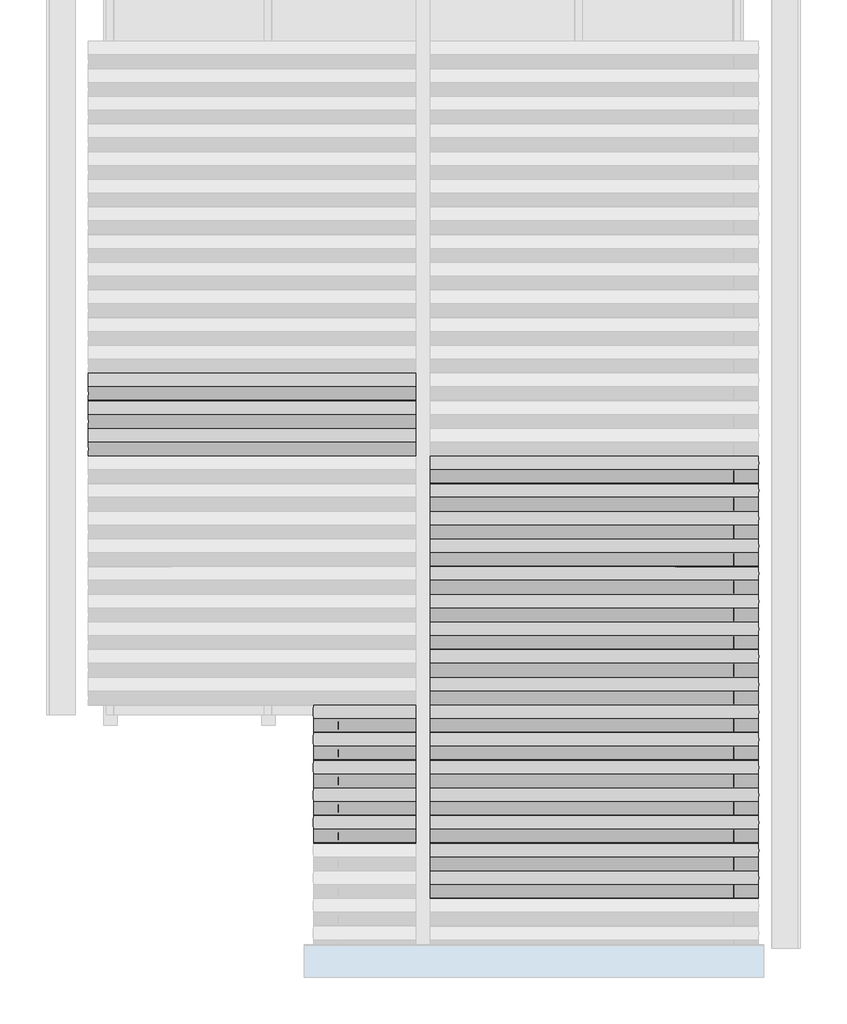
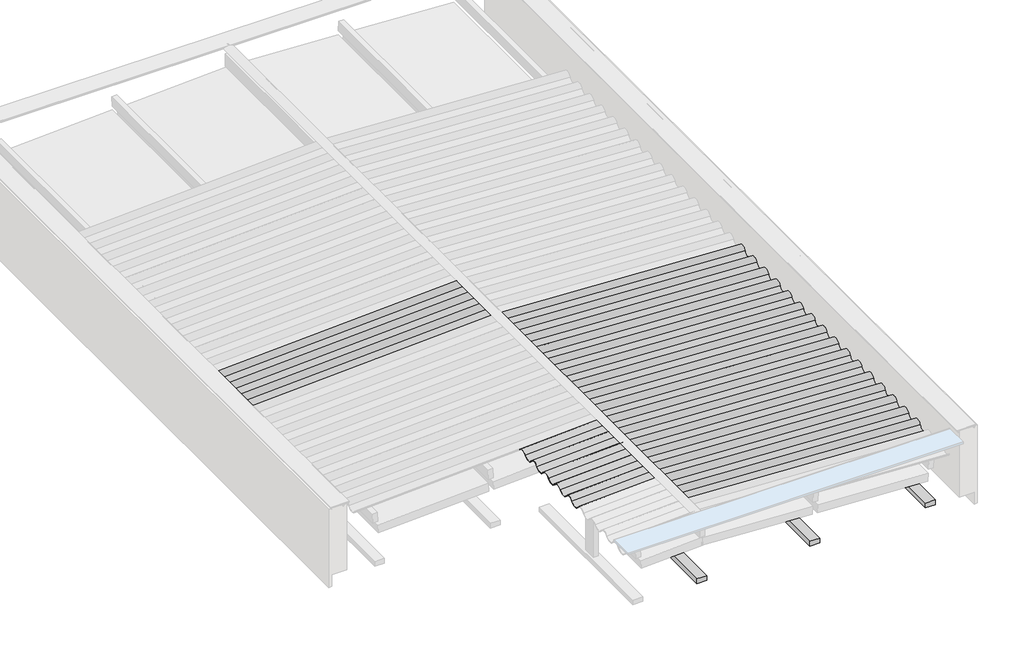
# One storey, part 2 of 4: 31 beams, 7 columns.
"""IFC4 building model written with IfcOpenShell, lengths in millimetres."""

import ifcopenshell
import ifcopenshell.guid

model = None  # the IFC model being written
_history = None  # IfcOwnerHistory: only IFC2X3 demands one
_inside = {}  # id of a spatial element -> (the spatial element, [elements in it])
_under = {}  # id of a project, library or spatial element -> (it, [spatial elements below it])
_declared = {}  # id of a project -> (the project, [libraries it declares])
_typed = {}  # id of a type object -> (the type object, [elements of that type])
_made_of = {}  # id of a material, layer set ... -> (it, [elements and type objects made of it])


def new_model(schema):
    """Start an empty IFC model of exactly this schema.

    Asked for "IFC4X3", IfcOpenShell would pick the latest addendum, in which some entities
    have other attributes; the version numbers below select the first issue.
    IFC2X3 requires an IfcOwnerHistory on every rooted entity: one is made here for all.
    """
    global model, _history
    if schema == "IFC4X3":
        model = ifcopenshell.file(schema_version=(4, 3, 0, 0))
    else:
        model = ifcopenshell.file(schema=schema)
    _inside.clear()
    _under.clear()
    _declared.clear()
    _typed.clear()
    _made_of.clear()
    _history = None
    if model.schema == "IFC2X3":
        org = make("IfcOrganization", Name="unknown")
        user = make(
            "IfcPersonAndOrganization",
            ThePerson=make("IfcPerson", FamilyName="unknown"),
            TheOrganization=org,
        )
        app = make(
            "IfcApplication",
            ApplicationDeveloper=org,
            Version="unknown",
            ApplicationFullName="unknown",
            ApplicationIdentifier="unknown",
        )
        _history = make(
            "IfcOwnerHistory",
            OwningUser=user,
            OwningApplication=app,
            ChangeAction="ADDED",
            CreationDate=0,
        )
    return model


def make(cls, **values):
    """One entity of the class cls with the attributes given. An attribute that is None is left unset."""
    return model.create_entity(
        cls, **{name: value for name, value in values.items() if value is not None}
    )


def rooted(cls, **values):
    """An entity with a GlobalId (a new one), such as an element, a storey or a relation."""
    return make(cls, GlobalId=ifcopenshell.guid.new(), OwnerHistory=_history, **values)


def si_unit(unit_type, name, prefix=None):
    """IfcSIUnit, for example si_unit("LENGTHUNIT", "METRE", prefix="MILLI")."""
    return make("IfcSIUnit", UnitType=unit_type, Prefix=prefix, Name=name)


def assignment(units):
    """IfcUnitAssignment: the units of a project."""
    return None if units is None else make("IfcUnitAssignment", Units=units)


def point(xyz):
    """IfcCartesianPoint."""
    return None if xyz is None else make("IfcCartesianPoint", Coordinates=xyz)


def direction(xyz):
    """IfcDirection."""
    return None if xyz is None else make("IfcDirection", DirectionRatios=xyz)


def frame(location, z_axis=None, x_axis=None):
    """IfcAxis2Placement3D, a coordinate frame: its origin and axes. An axis left out is left unset."""
    return make(
        "IfcAxis2Placement3D",
        Location=point(location),
        Axis=direction(z_axis),
        RefDirection=direction(x_axis),
    )


def frame_2d(location, x_axis=None):
    """IfcAxis2Placement2D, a coordinate frame in the plane: its origin and x axis."""
    return make(
        "IfcAxis2Placement2D", Location=point(location), RefDirection=direction(x_axis)
    )


def origin():
    """The frame at (0, 0, 0) with its axes left unset."""
    return frame((0.0, 0.0, 0.0))


def place(relative_to, where):
    """IfcLocalPlacement: puts the frame where relative to a parent placement (None: the world)."""
    return make(
        "IfcLocalPlacement", PlacementRelTo=relative_to, RelativePlacement=where
    )


def context(
    kind, dimensions, precision=None, world=None, true_north=None, identifier=None
):
    """IfcGeometricRepresentationContext, for example the 3D "Model" context."""
    return make(
        "IfcGeometricRepresentationContext",
        ContextIdentifier=identifier,
        ContextType=kind,
        CoordinateSpaceDimension=dimensions,
        Precision=precision,
        WorldCoordinateSystem=world,
        TrueNorth=true_north,
    )


def project(units=None, contexts=None):
    """IfcProject with its units and contexts."""
    return rooted(
        "IfcProject",
        Name="project",
        RepresentationContexts=contexts,
        UnitsInContext=assignment(units),
    )


def spatial(cls, under=None, at=None, **own):
    """A site, building, storey or space (cls), placed at a placement, below another one or the project."""
    s = rooted(cls, ObjectPlacement=at, **own)
    if under is not None:
        _under.setdefault(under.id(), (under, []))[1].append(s)
    return s


def polyline(points):
    """IfcPolyline through the points."""
    return make("IfcPolyline", Points=[point(p) for p in points])


def circle_curve(where, radius):
    """IfcCircle in the frame where."""
    return make("IfcCircle", Position=where, Radius=radius)


def trimmed(basis, trim1, trim2, sense, master):
    """IfcTrimmedCurve: the piece of a basis curve between two trims."""
    return make(
        "IfcTrimmedCurve",
        BasisCurve=basis,
        Trim1=trim1,
        Trim2=trim2,
        SenseAgreement=sense,
        MasterRepresentation=master,
    )


def segment(curve, same_sense, transition):
    """IfcCompositeCurveSegment."""
    return make(
        "IfcCompositeCurveSegment",
        Transition=transition,
        SameSense=same_sense,
        ParentCurve=curve,
    )


def composite_curve(segments, self_intersect=None):
    """IfcCompositeCurve: segments joined end to end."""
    return make("IfcCompositeCurve", Segments=segments, SelfIntersect=self_intersect)


def outline(outer, holes=None, kind="AREA"):
    """IfcArbitraryClosedProfileDef: a profile drawn as a closed curve; with holes, ...WithVoids."""
    if holes is None:
        return make("IfcArbitraryClosedProfileDef", ProfileType=kind, OuterCurve=outer)
    return make(
        "IfcArbitraryProfileDefWithVoids",
        ProfileType=kind,
        OuterCurve=outer,
        InnerCurves=holes,
    )


def extrude(swept, where, along, depth):
    """IfcExtrudedAreaSolid: the profile swept, set in the frame where, extruded along a direction by depth."""
    return make(
        "IfcExtrudedAreaSolid",
        SweptArea=swept,
        Position=where,
        ExtrudedDirection=direction(along),
        Depth=depth,
    )


def shape(context_of_items, identifier, shape_type, items):
    """IfcShapeRepresentation: the items that make up one representation, for example the "Body"."""
    return make(
        "IfcShapeRepresentation",
        ContextOfItems=context_of_items,
        RepresentationIdentifier=identifier,
        RepresentationType=shape_type,
        Items=items,
    )


def source(mapping_origin, context_of_items, identifier, shape_type, items):
    """IfcRepresentationMap: a shape defined once, which mapped items show again and again."""
    return make(
        "IfcRepresentationMap",
        MappingOrigin=mapping_origin,
        MappedRepresentation=shape(context_of_items, identifier, shape_type, items),
    )


def transform(
    local_origin,
    x_axis=None,
    y_axis=None,
    z_axis=None,
    scale=None,
    scale2=None,
    scale3=None,
    uniform=True,
):
    """IfcCartesianTransformationOperator3D, or its non-uniform kind. x_axis, y_axis, z_axis: its Axis1, 2, 3."""
    if uniform:
        return make(
            "IfcCartesianTransformationOperator3D",
            Axis1=direction(x_axis),
            Axis2=direction(y_axis),
            LocalOrigin=point(local_origin),
            Scale=scale,
            Axis3=direction(z_axis),
        )
    return make(
        "IfcCartesianTransformationOperator3DnonUniform",
        Axis1=direction(x_axis),
        Axis2=direction(y_axis),
        LocalOrigin=point(local_origin),
        Scale=scale,
        Axis3=direction(z_axis),
        Scale2=scale2,
        Scale3=scale3,
    )


def mapped(mapping_source, mapping_target):
    """IfcMappedItem: shows the shape of a source again, moved by a transform."""
    return make(
        "IfcMappedItem", MappingSource=mapping_source, MappingTarget=mapping_target
    )


def made_of(thing, what):
    """Note that an element or type object is made of a material, layer set ...; save() writes the relation."""
    if what is not None:
        _made_of.setdefault(what.id(), (what, []))[1].append(thing)
    return thing


def element(
    cls,
    number,
    at=None,
    inside=None,
    cuts=None,
    type_object=None,
    material=None,
    context=None,
    identifier="Body",
    shape_type=None,
    held_by="IfcProductDefinitionShape",
    body=None,
    shapes=None,
    **own,
):
    """One element of the class cls, such as IfcWall. Its Tag is "e" and its number.

    at: its placement. inside: the storey or other place that contains it. cuts: it is an
    opening in that element (IfcRelVoidsElement). A single representation is given by context,
    identifier, shape_type and body (its items); several are given by shapes. held_by: the class
    of the entity that holds the representations. save() writes the other relations.
    """
    e = rooted(cls, Tag="e%d" % number, ObjectPlacement=at, **own)
    if body is not None:
        shapes = [shape(context, identifier, shape_type, body)]
    if shapes is not None:
        e.Representation = make(held_by, Representations=shapes)
    if inside is not None:
        _inside.setdefault(inside.id(), (inside, []))[1].append(e)
    if cuts is not None:
        rooted(
            "IfcRelVoidsElement", RelatingBuildingElement=cuts, RelatedOpeningElement=e
        )
    if type_object is not None:
        _typed.setdefault(type_object.id(), (type_object, []))[1].append(e)
    return made_of(e, material)


def aggregate(whole, parts):
    """IfcRelAggregates: a whole, such as a stair, and the parts it consists of."""
    return rooted("IfcRelAggregates", RelatingObject=whole, RelatedObjects=parts)


def save(model, path):
    """Write the relations noted so far, then the file.

    IfcRelAggregates (storeys below a building ...), IfcRelContainedInSpatialStructure (elements
    in a storey), IfcRelDefinesByType, IfcRelAssociatesMaterial and IfcRelDeclares: one each for
    every whole, place, type object, material and project.
    """
    for whole, parts in _under.values():
        aggregate(whole, parts)
    for where, things in _inside.values():
        rooted(
            "IfcRelContainedInSpatialStructure",
            RelatedElements=things,
            RelatingStructure=where,
        )
    for kind, things in _typed.values():
        rooted("IfcRelDefinesByType", RelatedObjects=things, RelatingType=kind)
    for what, things in _made_of.values():
        rooted("IfcRelAssociatesMaterial", RelatedObjects=things, RelatingMaterial=what)
    for by, libraries in _declared.values():
        rooted("IfcRelDeclares", RelatingContext=by, RelatedDefinitions=libraries)
    model.write(path)


def column_f3930958(model_context):
    return source(origin(), model_context, "Body", "SweptSolid", [
        extrude(outline(polyline([(30.0, 80.0), (30.0, -80.0), (-30.0, -80.0), (-30.0, 80.0), (30.0, 80.0)])), frame((0.0, 0.0, 4460.0), z_axis=(0.0, 0.0, 1.0), x_axis=(1.0, 0.0, 0.0)), (0.0, 0.0, 1.0), 522.9),
    ])


def column_4d3918cc(model_context):
    return source(origin(), model_context, "Body", "SweptSolid", [
        extrude(outline(polyline([(30.0, 80.0), (30.0, -80.0), (-30.0, -80.0), (-30.0, 80.0), (30.0, 80.0)])), frame((0.0, 0.0, 4460.0), z_axis=(0.0, 0.0, 1.0), x_axis=(1.0, 0.0, 0.0)), (0.0, 0.0, 1.0), 426.9),
    ])


def column_924cc83b(model_context):
    return source(origin(), model_context, "Body", "SweptSolid", [
        extrude(outline(polyline([(30.0, 80.0), (30.0, -80.0), (-30.0, -80.0), (-30.0, 80.0), (30.0, 80.0)])), frame((0.0, 0.0, 4460.0), z_axis=(0.0, 0.0, 1.0), x_axis=(1.0, 0.0, 0.0)), (0.0, 0.0, 1.0), 497.0),
    ])


model = new_model("IFC4")

# Units and contexts
model_context = context("Model", 3, world=origin())
ifc_project = project(units=[si_unit("LENGTHUNIT", "METRE", prefix="MILLI")], contexts=[model_context])

# Site, building, storey
site = spatial("IfcSite", under=ifc_project)
building = spatial("IfcBuilding", under=site)
storey = spatial("IfcBuildingStorey", under=building, Name="COB. SALA ESTAR", Elevation=4400.0)

# Beams
placement = place(None, origin())
element("IfcBeam", 1, ObjectType="Madeira de lei : Berço 6x12cm", at=placement, inside=storey, context=model_context, shape_type="SweptSolid", body=[
    extrude(outline(polyline([(-3400.781307, -376.0699847), (-3280.781307, -376.0699847), (-3280.781307, -2376.0699847), (-3400.781307, -2376.0699847), (-3400.781307, -376.0699847)])), frame((0.0, 0.0, 4400.0), z_axis=(0.0, 0.0, 1.0), x_axis=(1.0, 0.0, 0.0)), (0.0, 0.0, 1.0), 60.0),
])
element("IfcBeam", 2, ObjectType="Madeira de lei : Berço 6x12cm", at=placement, inside=storey, context=model_context, shape_type="SweptSolid", body=[
    extrude(outline(polyline([(-3400.781307, -2376.0699847), (-3280.781307, -2376.0699847), (-3280.781307, -4336.0699847), (-3400.781307, -4336.0699847), (-3400.781307, -2376.0699847)])), frame((0.0, 0.0, 4400.0), z_axis=(0.0, 0.0, 1.0), x_axis=(1.0, 0.0, 0.0)), (0.0, 0.0, 1.0), 60.0),
])
element("IfcBeam", 3, ObjectType="Madeira de lei : Berço 6x12cm", at=placement, inside=storey, context=model_context, shape_type="SweptSolid", body=[
    extrude(outline(polyline([(-2032.4438771, -376.0699847), (-1912.4438771, -376.0699847), (-1912.4438771, -2376.0699847), (-2032.4438771, -2376.0699847), (-2032.4438771, -376.0699847)])), frame((0.0, 0.0, 4400.0), z_axis=(0.0, 0.0, 1.0), x_axis=(1.0, 0.0, 0.0)), (0.0, 0.0, 1.0), 60.0),
])
element("IfcBeam", 4, ObjectType="Madeira de lei : Berço 6x12cm", at=placement, inside=storey, context=model_context, shape_type="SweptSolid", body=[
    extrude(outline(polyline([(-2032.4438771, -2376.0699847), (-1912.4438771, -2376.0699847), (-1912.4438771, -4336.0699847), (-2032.4438771, -4336.0699847), (-2032.4438771, -2376.0699847)])), frame((0.0, 0.0, 4400.0), z_axis=(0.0, 0.0, 1.0), x_axis=(1.0, 0.0, 0.0)), (0.0, 0.0, 1.0), 60.0),
])
element("IfcBeam", 5, ObjectType="Madeira de lei : Berço 6x12cm", at=placement, inside=storey, context=model_context, shape_type="SweptSolid", body=[
    extrude(outline(polyline([(-634.1438771, -376.0699847), (-514.1438771, -376.0699847), (-514.1438771, -2376.0699847), (-634.1438771, -2376.0699847), (-634.1438771, -376.0699847)])), frame((0.0, 0.0, 4400.0), z_axis=(0.0, 0.0, 1.0), x_axis=(1.0, 0.0, 0.0)), (0.0, 0.0, 1.0), 60.0),
])
element("IfcBeam", 6, ObjectType="Madeira de lei : Berço 6x12cm", at=placement, inside=storey, context=model_context, shape_type="SweptSolid", body=[
    extrude(outline(polyline([(-634.1438771, -2376.0699847), (-514.1438771, -2376.0699847), (-514.1438771, -4336.0699847), (-634.1438771, -4336.0699847), (-634.1438771, -2376.0699847)])), frame((0.0, 0.0, 4400.0), z_axis=(0.0, 0.0, 1.0), x_axis=(1.0, 0.0, 0.0)), (0.0, 0.0, 1.0), 60.0),
])
element("IfcBeam", 7, ObjectType="Madeira de lei : Berço 6x12cm", at=placement, inside=storey, context=model_context, shape_type="SweptSolid", body=[
    extrude(outline(polyline([(-6167.4187368, 1623.9300153), (-6047.4187368, 1623.9300153), (-6047.4187368, -376.0699847), (-6167.4187368, -376.0699847), (-6167.4187368, 1623.9300153)])), frame((0.0, 0.0, 4400.0), z_axis=(0.0, 0.0, 1.0), x_axis=(1.0, 0.0, 0.0)), (0.0, 0.0, 1.0), 60.0),
])
element("IfcBeam", 8, ObjectType="Telha Ondulada : Fibrocimento", at=placement, inside=storey, context=model_context, shape_type="SweptSolid", body=[
    extrude(outline(composite_curve([segment(trimmed(circle_curve(frame_2d((-58.7002978, -53.2060538)), 66.7939461), [point((-29.3501489, 6.7939462))], [point((-29.3501489, -113.2060538))], False, "CARTESIAN"), True, "CONTINUOUS"), segment(polyline([(-29.3501489, -113.2060538), (-31.5472154, -108.7146288)]), True, "CONTINUOUS"), segment(trimmed(circle_curve(frame_2d((-58.7002978, -53.2060538)), 61.7939461), [point((-31.5472154, -108.7146288))], [point((-31.5472154, 2.3025211))], True, "CARTESIAN"), True, "CONTINUOUS"), segment(trimmed(circle_curve(frame_2d((0.0, 66.7939462)), 71.7939461), [point((-31.5472154, 2.3025211))], [point((-31.5472154, 131.2853712))], False, "CARTESIAN"), True, "CONTINUOUS"), segment(polyline([(-31.5472154, 131.2853712), (-29.3501489, 126.7939462)]), True, "CONTINUOUS"), segment(trimmed(circle_curve(frame_2d((0.0, 66.7939462)), 66.7939461), [point((-29.3501489, 126.7939462))], [point((-29.3501489, 6.7939462))], True, "CARTESIAN"), True, "CONTINUOUS")], self_intersect=False)), frame((-4311.894473, -3289.673052, 5167.7128806), z_axis=(0.9987523388778448, 0.0, 0.049937616943891816), x_axis=(-0.049937616943891816, 0.0, 0.9987523388778448)), (0.0, 0.0, 1.0), 967.7366024),
])
element("IfcBeam", 9, ObjectType="Telha Ondulada : Fibrocimento", at=placement, inside=storey, context=model_context, shape_type="SweptSolid", body=[
    extrude(outline(composite_curve([segment(trimmed(circle_curve(frame_2d((-58.7002978, -53.2060538)), 66.7939461), [point((-29.3501489, 6.7939462))], [point((-29.3501489, -113.2060538))], False, "CARTESIAN"), True, "CONTINUOUS"), segment(polyline([(-29.3501489, -113.2060538), (-31.5472154, -108.7146288)]), True, "CONTINUOUS"), segment(trimmed(circle_curve(frame_2d((-58.7002978, -53.2060538)), 61.7939461), [point((-31.5472154, -108.7146288))], [point((-31.5472154, 2.3025211))], True, "CARTESIAN"), True, "CONTINUOUS"), segment(trimmed(circle_curve(frame_2d((0.0, 66.7939462)), 71.7939461), [point((-31.5472154, 2.3025211))], [point((-31.5472154, 131.2853712))], False, "CARTESIAN"), True, "CONTINUOUS"), segment(polyline([(-31.5472154, 131.2853712), (-29.3501489, 126.7939462)]), True, "CONTINUOUS"), segment(trimmed(circle_curve(frame_2d((0.0, 66.7939462)), 66.7939461), [point((-29.3501489, 126.7939462))], [point((-29.3501489, 6.7939462))], True, "CARTESIAN"), True, "CONTINUOUS")], self_intersect=False)), frame((-4311.894473, -3045.173052, 5167.7128806), z_axis=(0.9987523388778448, 0.0, 0.049937616943891816), x_axis=(-0.049937616943891816, 0.0, 0.9987523388778448)), (0.0, 0.0, 1.0), 967.7366024),
])
element("IfcBeam", 10, ObjectType="Telha Ondulada : Fibrocimento", at=placement, inside=storey, context=model_context, shape_type="SweptSolid", body=[
    extrude(outline(composite_curve([segment(trimmed(circle_curve(frame_2d((-58.7002978, -53.2060538)), 66.7939461), [point((-29.3501489, 6.7939462))], [point((-29.3501489, -113.2060538))], False, "CARTESIAN"), True, "CONTINUOUS"), segment(polyline([(-29.3501489, -113.2060538), (-31.5472154, -108.7146288)]), True, "CONTINUOUS"), segment(trimmed(circle_curve(frame_2d((-58.7002978, -53.2060538)), 61.7939461), [point((-31.5472154, -108.7146288))], [point((-31.5472154, 2.3025211))], True, "CARTESIAN"), True, "CONTINUOUS"), segment(trimmed(circle_curve(frame_2d((0.0, 66.7939462)), 71.7939461), [point((-31.5472154, 2.3025211))], [point((-31.5472154, 131.2853712))], False, "CARTESIAN"), True, "CONTINUOUS"), segment(polyline([(-31.5472154, 131.2853712), (-29.3501489, 126.7939462)]), True, "CONTINUOUS"), segment(trimmed(circle_curve(frame_2d((0.0, 66.7939462)), 66.7939461), [point((-29.3501489, 126.7939462))], [point((-29.3501489, 6.7939462))], True, "CARTESIAN"), True, "CONTINUOUS")], self_intersect=False)), frame((-4311.894473, -2800.673052, 5167.7128806), z_axis=(0.9987523388778448, 0.0, 0.049937616943891844), x_axis=(-0.049937616943891844, 0.0, 0.9987523388778448)), (0.0, 0.0, 1.0), 967.7366024),
])
element("IfcBeam", 11, ObjectType="Telha Ondulada : Fibrocimento", at=placement, inside=storey, context=model_context, shape_type="SweptSolid", body=[
    extrude(outline(composite_curve([segment(trimmed(circle_curve(frame_2d((-58.7002978, -53.2060538)), 66.7939461), [point((-29.3501489, 6.7939462))], [point((-29.3501489, -113.2060538))], False, "CARTESIAN"), True, "CONTINUOUS"), segment(polyline([(-29.3501489, -113.2060538), (-31.5472154, -108.7146288)]), True, "CONTINUOUS"), segment(trimmed(circle_curve(frame_2d((-58.7002978, -53.2060538)), 61.7939461), [point((-31.5472154, -108.7146288))], [point((-31.5472154, 2.3025211))], True, "CARTESIAN"), True, "CONTINUOUS"), segment(trimmed(circle_curve(frame_2d((0.0, 66.7939462)), 71.7939461), [point((-31.5472154, 2.3025211))], [point((-31.5472154, 131.2853712))], False, "CARTESIAN"), True, "CONTINUOUS"), segment(polyline([(-31.5472154, 131.2853712), (-29.3501489, 126.7939462)]), True, "CONTINUOUS"), segment(trimmed(circle_curve(frame_2d((0.0, 66.7939462)), 66.7939461), [point((-29.3501489, 126.7939462))], [point((-29.3501489, 6.7939462))], True, "CARTESIAN"), True, "CONTINUOUS")], self_intersect=False)), frame((-4311.894473, -2556.173052, 5167.7128806), z_axis=(0.9987523388778448, 0.0, 0.049937616943891816), x_axis=(-0.049937616943891816, 0.0, 0.9987523388778448)), (0.0, 0.0, 1.0), 967.7366024),
])
element("IfcBeam", 12, ObjectType="Telha Ondulada : Fibrocimento", at=placement, inside=storey, context=model_context, shape_type="SweptSolid", body=[
    extrude(outline(composite_curve([segment(trimmed(circle_curve(frame_2d((-58.7002978, -53.2060538)), 66.7939461), [point((-29.3501489, 6.7939462))], [point((-29.3501489, -113.2060538))], False, "CARTESIAN"), True, "CONTINUOUS"), segment(polyline([(-29.3501489, -113.2060538), (-31.5472154, -108.7146288)]), True, "CONTINUOUS"), segment(trimmed(circle_curve(frame_2d((-58.7002978, -53.2060538)), 61.7939461), [point((-31.5472154, -108.7146288))], [point((-31.5472154, 2.3025211))], True, "CARTESIAN"), True, "CONTINUOUS"), segment(trimmed(circle_curve(frame_2d((0.0, 66.7939462)), 71.7939461), [point((-31.5472154, 2.3025211))], [point((-31.5472154, 131.2853712))], False, "CARTESIAN"), True, "CONTINUOUS"), segment(polyline([(-31.5472154, 131.2853712), (-29.3501489, 126.7939462)]), True, "CONTINUOUS"), segment(trimmed(circle_curve(frame_2d((0.0, 66.7939462)), 66.7939461), [point((-29.3501489, 126.7939462))], [point((-29.3501489, 6.7939462))], True, "CARTESIAN"), True, "CONTINUOUS")], self_intersect=False)), frame((-4311.894473, -2311.673052, 5167.7128806), z_axis=(0.9987523388778448, 0.0, 0.04993761694389179), x_axis=(-0.04993761694389179, 0.0, 0.9987523388778448)), (0.0, 0.0, 1.0), 967.7366024),
])
element("IfcBeam", 13, ObjectType="Telha Ondulada : Fibrocimento", at=placement, inside=storey, context=model_context, shape_type="SweptSolid", body=[
    extrude(outline(composite_curve([segment(trimmed(circle_curve(frame_2d((-58.7002978, -53.2060538)), 66.7939461), [point((-29.3501488, 6.7939462))], [point((-29.3501488, -113.2060538))], False, "CARTESIAN"), True, "CONTINUOUS"), segment(polyline([(-29.3501488, -113.2060538), (-31.5472154, -108.7146288)]), True, "CONTINUOUS"), segment(trimmed(circle_curve(frame_2d((-58.7002978, -53.2060538)), 61.7939461), [point((-31.5472154, -108.7146288))], [point((-31.5472154, 2.3025211))], True, "CARTESIAN"), True, "CONTINUOUS"), segment(trimmed(circle_curve(frame_2d((0.0, 66.7939462)), 71.7939461), [point((-31.5472154, 2.3025211))], [point((-31.5472154, 131.2853712))], False, "CARTESIAN"), True, "CONTINUOUS"), segment(polyline([(-31.5472154, 131.2853712), (-29.3501488, 126.7939462)]), True, "CONTINUOUS"), segment(trimmed(circle_curve(frame_2d((0.0, 66.7939462)), 66.7939461), [point((-29.3501488, 126.7939462))], [point((-29.3501488, 6.7939462))], True, "CARTESIAN"), True, "CONTINUOUS")], self_intersect=False)), frame((-6303.6781287, 133.326948, 5068.1236978), z_axis=(0.9987523388778448, 0.0, 0.049937616943891344), x_axis=(-0.049937616943891344, 0.0, 0.9987523388778448)), (0.0, 0.0, 1.0), 2962.0084336),
])
element("IfcBeam", 14, ObjectType="Telha Ondulada : Fibrocimento", at=placement, inside=storey, context=model_context, shape_type="SweptSolid", body=[
    extrude(outline(composite_curve([segment(trimmed(circle_curve(frame_2d((-58.7002978, -53.2060538)), 66.7939461), [point((-29.3501488, 6.7939462))], [point((-29.3501488, -113.2060538))], False, "CARTESIAN"), True, "CONTINUOUS"), segment(polyline([(-29.3501488, -113.2060538), (-31.5472154, -108.7146288)]), True, "CONTINUOUS"), segment(trimmed(circle_curve(frame_2d((-58.7002978, -53.2060538)), 61.7939461), [point((-31.5472154, -108.7146288))], [point((-31.5472154, 2.3025211))], True, "CARTESIAN"), True, "CONTINUOUS"), segment(trimmed(circle_curve(frame_2d((0.0, 66.7939462)), 71.7939461), [point((-31.5472154, 2.3025211))], [point((-31.5472154, 131.2853712))], False, "CARTESIAN"), True, "CONTINUOUS"), segment(polyline([(-31.5472154, 131.2853712), (-29.3501488, 126.7939462)]), True, "CONTINUOUS"), segment(trimmed(circle_curve(frame_2d((0.0, 66.7939462)), 66.7939461), [point((-29.3501488, 126.7939462))], [point((-29.3501488, 6.7939462))], True, "CARTESIAN"), True, "CONTINUOUS")], self_intersect=False)), frame((-6303.6781287, 377.826948, 5068.1236978), z_axis=(0.9987523388778449, 0.0, 0.049937616943891365), x_axis=(-0.049937616943891365, 0.0, 0.9987523388778449)), (0.0, 0.0, 1.0), 2962.0084336),
])
element("IfcBeam", 15, ObjectType="Telha Ondulada : Fibrocimento", at=placement, inside=storey, context=model_context, shape_type="SweptSolid", body=[
    extrude(outline(composite_curve([segment(trimmed(circle_curve(frame_2d((-58.7002978, -53.2060538)), 66.7939461), [point((-29.3501488, 6.7939462))], [point((-29.3501488, -113.2060538))], False, "CARTESIAN"), True, "CONTINUOUS"), segment(polyline([(-29.3501488, -113.2060538), (-31.5472154, -108.7146288)]), True, "CONTINUOUS"), segment(trimmed(circle_curve(frame_2d((-58.7002978, -53.2060538)), 61.7939461), [point((-31.5472154, -108.7146288))], [point((-31.5472154, 2.3025211))], True, "CARTESIAN"), True, "CONTINUOUS"), segment(trimmed(circle_curve(frame_2d((0.0, 66.7939462)), 71.7939461), [point((-31.5472154, 2.3025211))], [point((-31.5472154, 131.2853712))], False, "CARTESIAN"), True, "CONTINUOUS"), segment(polyline([(-31.5472154, 131.2853712), (-29.3501488, 126.7939462)]), True, "CONTINUOUS"), segment(trimmed(circle_curve(frame_2d((0.0, 66.7939462)), 66.7939461), [point((-29.3501488, 126.7939462))], [point((-29.3501488, 6.7939462))], True, "CARTESIAN"), True, "CONTINUOUS")], self_intersect=False)), frame((-6303.6781287, 622.326948, 5068.1236978), z_axis=(0.9987523388778448, 0.0, 0.04993761694389136), x_axis=(-0.04993761694389136, 0.0, 0.9987523388778448)), (0.0, 0.0, 1.0), 2962.0084336),
])
element("IfcBeam", 16, ObjectType="Telha Ondulada : Fibrocimento", at=placement, inside=storey, context=model_context, shape_type="SweptSolid", body=[
    extrude(outline(composite_curve([segment(trimmed(circle_curve(frame_2d((0.0, 66.7939462)), 66.7939461), [point((29.3501488, 6.7939462))], [point((29.3501488, 126.7939462))], True, "CARTESIAN"), True, "CONTINUOUS"), segment(polyline([(29.3501488, 126.7939462), (31.5472154, 131.2853712)]), True, "CONTINUOUS"), segment(trimmed(circle_curve(frame_2d((0.0, 66.7939462)), 71.7939461), [point((31.5472154, 131.2853712))], [point((31.5472154, 2.3025211))], False, "CARTESIAN"), True, "CONTINUOUS"), segment(trimmed(circle_curve(frame_2d((58.7002978, -53.2060538)), 61.7939461), [point((31.5472154, 2.3025211))], [point((31.5472154, -108.7146288))], True, "CARTESIAN"), True, "CONTINUOUS"), segment(polyline([(31.5472154, -108.7146288), (29.3501488, -113.2060538)]), True, "CONTINUOUS"), segment(trimmed(circle_curve(frame_2d((58.7002978, -53.2060538)), 66.7939461), [point((29.3501488, -113.2060538))], [point((29.3501488, 6.7939462))], False, "CARTESIAN"), True, "CONTINUOUS")], self_intersect=False)), frame((-377.8844852, -3778.673052, 5068.1236978), z_axis=(-0.9987523388778448, 0.0, 0.049937616943891455), x_axis=(-0.049937616943891455, 0.0, -0.9987523388778448)), (0.0, 0.0, 1.0), 2962.0084336),
])
element("IfcBeam", 17, ObjectType="Telha Ondulada : Fibrocimento", at=placement, inside=storey, context=model_context, shape_type="SweptSolid", body=[
    extrude(outline(composite_curve([segment(trimmed(circle_curve(frame_2d((0.0, 66.7939462)), 66.7939461), [point((29.3501488, 6.7939462))], [point((29.3501488, 126.7939462))], True, "CARTESIAN"), True, "CONTINUOUS"), segment(polyline([(29.3501488, 126.7939462), (31.5472154, 131.2853712)]), True, "CONTINUOUS"), segment(trimmed(circle_curve(frame_2d((0.0, 66.7939462)), 71.7939461), [point((31.5472154, 131.2853712))], [point((31.5472154, 2.3025211))], False, "CARTESIAN"), True, "CONTINUOUS"), segment(trimmed(circle_curve(frame_2d((58.7002978, -53.2060538)), 61.7939461), [point((31.5472154, 2.3025211))], [point((31.5472154, -108.7146288))], True, "CARTESIAN"), True, "CONTINUOUS"), segment(polyline([(31.5472154, -108.7146288), (29.3501488, -113.2060538)]), True, "CONTINUOUS"), segment(trimmed(circle_curve(frame_2d((58.7002978, -53.2060538)), 66.7939461), [point((29.3501488, -113.2060538))], [point((29.3501488, 6.7939462))], False, "CARTESIAN"), True, "CONTINUOUS")], self_intersect=False)), frame((-377.8844852, -3534.173052, 5068.1236978), z_axis=(-0.9987523388778448, 0.0, 0.049937616943891455), x_axis=(-0.049937616943891455, 0.0, -0.9987523388778448)), (0.0, 0.0, 1.0), 2962.0084336),
])
element("IfcBeam", 18, ObjectType="Telha Ondulada : Fibrocimento", at=placement, inside=storey, context=model_context, shape_type="SweptSolid", body=[
    extrude(outline(composite_curve([segment(trimmed(circle_curve(frame_2d((0.0, 66.7939462)), 66.7939461), [point((29.3501488, 6.7939462))], [point((29.3501488, 126.7939462))], True, "CARTESIAN"), True, "CONTINUOUS"), segment(polyline([(29.3501488, 126.7939462), (31.5472154, 131.2853712)]), True, "CONTINUOUS"), segment(trimmed(circle_curve(frame_2d((0.0, 66.7939462)), 71.7939461), [point((31.5472154, 131.2853712))], [point((31.5472154, 2.3025211))], False, "CARTESIAN"), True, "CONTINUOUS"), segment(trimmed(circle_curve(frame_2d((58.7002978, -53.2060538)), 61.7939461), [point((31.5472154, 2.3025211))], [point((31.5472154, -108.7146288))], True, "CARTESIAN"), True, "CONTINUOUS"), segment(polyline([(31.5472154, -108.7146288), (29.3501488, -113.2060538)]), True, "CONTINUOUS"), segment(trimmed(circle_curve(frame_2d((58.7002978, -53.2060538)), 66.7939461), [point((29.3501488, -113.2060538))], [point((29.3501488, 6.7939462))], False, "CARTESIAN"), True, "CONTINUOUS")], self_intersect=False)), frame((-377.8844852, -3289.673052, 5068.1236978), z_axis=(-0.9987523388778448, 0.0, 0.049937616943891455), x_axis=(-0.049937616943891455, 0.0, -0.9987523388778448)), (0.0, 0.0, 1.0), 2962.0084336),
])
element("IfcBeam", 19, ObjectType="Telha Ondulada : Fibrocimento", at=placement, inside=storey, context=model_context, shape_type="SweptSolid", body=[
    extrude(outline(composite_curve([segment(trimmed(circle_curve(frame_2d((0.0, 66.7939462)), 66.7939461), [point((29.3501488, 6.7939462))], [point((29.3501488, 126.7939462))], True, "CARTESIAN"), True, "CONTINUOUS"), segment(polyline([(29.3501488, 126.7939462), (31.5472154, 131.2853712)]), True, "CONTINUOUS"), segment(trimmed(circle_curve(frame_2d((0.0, 66.7939462)), 71.7939461), [point((31.5472154, 131.2853712))], [point((31.5472154, 2.3025211))], False, "CARTESIAN"), True, "CONTINUOUS"), segment(trimmed(circle_curve(frame_2d((58.7002978, -53.2060538)), 61.7939461), [point((31.5472154, 2.3025211))], [point((31.5472154, -108.7146288))], True, "CARTESIAN"), True, "CONTINUOUS"), segment(polyline([(31.5472154, -108.7146288), (29.3501488, -113.2060538)]), True, "CONTINUOUS"), segment(trimmed(circle_curve(frame_2d((58.7002978, -53.2060538)), 66.7939461), [point((29.3501488, -113.2060538))], [point((29.3501488, 6.7939462))], False, "CARTESIAN"), True, "CONTINUOUS")], self_intersect=False)), frame((-377.8844852, -3045.173052, 5068.1236978), z_axis=(-0.9987523388778448, 0.0, 0.049937616943891455), x_axis=(-0.049937616943891455, 0.0, -0.9987523388778448)), (0.0, 0.0, 1.0), 2962.0084336),
])
element("IfcBeam", 20, ObjectType="Telha Ondulada : Fibrocimento", at=placement, inside=storey, context=model_context, shape_type="SweptSolid", body=[
    extrude(outline(composite_curve([segment(trimmed(circle_curve(frame_2d((0.0, 66.7939462)), 66.7939461), [point((29.3501488, 6.7939462))], [point((29.3501488, 126.7939462))], True, "CARTESIAN"), True, "CONTINUOUS"), segment(polyline([(29.3501488, 126.7939462), (31.5472154, 131.2853712)]), True, "CONTINUOUS"), segment(trimmed(circle_curve(frame_2d((0.0, 66.7939462)), 71.7939461), [point((31.5472154, 131.2853712))], [point((31.5472154, 2.3025211))], False, "CARTESIAN"), True, "CONTINUOUS"), segment(trimmed(circle_curve(frame_2d((58.7002978, -53.2060538)), 61.7939461), [point((31.5472154, 2.3025211))], [point((31.5472154, -108.7146288))], True, "CARTESIAN"), True, "CONTINUOUS"), segment(polyline([(31.5472154, -108.7146288), (29.3501488, -113.2060538)]), True, "CONTINUOUS"), segment(trimmed(circle_curve(frame_2d((58.7002978, -53.2060538)), 66.7939461), [point((29.3501488, -113.2060538))], [point((29.3501488, 6.7939462))], False, "CARTESIAN"), True, "CONTINUOUS")], self_intersect=False)), frame((-377.8844852, -2800.673052, 5068.1236978), z_axis=(-0.9987523388778448, 0.0, 0.049937616943891455), x_axis=(-0.049937616943891455, 0.0, -0.9987523388778448)), (0.0, 0.0, 1.0), 2962.0084336),
])
element("IfcBeam", 21, ObjectType="Telha Ondulada : Fibrocimento", at=placement, inside=storey, context=model_context, shape_type="SweptSolid", body=[
    extrude(outline(composite_curve([segment(trimmed(circle_curve(frame_2d((0.0, 66.7939462)), 66.7939461), [point((29.3501488, 6.7939462))], [point((29.3501488, 126.7939462))], True, "CARTESIAN"), True, "CONTINUOUS"), segment(polyline([(29.3501488, 126.7939462), (31.5472154, 131.2853712)]), True, "CONTINUOUS"), segment(trimmed(circle_curve(frame_2d((0.0, 66.7939462)), 71.7939461), [point((31.5472154, 131.2853712))], [point((31.5472154, 2.3025211))], False, "CARTESIAN"), True, "CONTINUOUS"), segment(trimmed(circle_curve(frame_2d((58.7002978, -53.2060538)), 61.7939461), [point((31.5472154, 2.3025211))], [point((31.5472154, -108.7146288))], True, "CARTESIAN"), True, "CONTINUOUS"), segment(polyline([(31.5472154, -108.7146288), (29.3501488, -113.2060538)]), True, "CONTINUOUS"), segment(trimmed(circle_curve(frame_2d((58.7002978, -53.2060538)), 66.7939461), [point((29.3501488, -113.2060538))], [point((29.3501488, 6.7939462))], False, "CARTESIAN"), True, "CONTINUOUS")], self_intersect=False)), frame((-377.8844852, -2556.173052, 5068.1236978), z_axis=(-0.9987523388778448, 0.0, 0.049937616943891455), x_axis=(-0.049937616943891455, 0.0, -0.9987523388778448)), (0.0, 0.0, 1.0), 2962.0084336),
])
element("IfcBeam", 22, ObjectType="Telha Ondulada : Fibrocimento", at=placement, inside=storey, context=model_context, shape_type="SweptSolid", body=[
    extrude(outline(composite_curve([segment(trimmed(circle_curve(frame_2d((0.0, 66.7939462)), 66.7939461), [point((29.3501488, 6.7939462))], [point((29.3501488, 126.7939462))], True, "CARTESIAN"), True, "CONTINUOUS"), segment(polyline([(29.3501488, 126.7939462), (31.5472154, 131.2853712)]), True, "CONTINUOUS"), segment(trimmed(circle_curve(frame_2d((0.0, 66.7939462)), 71.7939461), [point((31.5472154, 131.2853712))], [point((31.5472154, 2.3025211))], False, "CARTESIAN"), True, "CONTINUOUS"), segment(trimmed(circle_curve(frame_2d((58.7002978, -53.2060538)), 61.7939461), [point((31.5472154, 2.3025211))], [point((31.5472154, -108.7146288))], True, "CARTESIAN"), True, "CONTINUOUS"), segment(polyline([(31.5472154, -108.7146288), (29.3501488, -113.2060538)]), True, "CONTINUOUS"), segment(trimmed(circle_curve(frame_2d((58.7002978, -53.2060538)), 66.7939461), [point((29.3501488, -113.2060538))], [point((29.3501488, 6.7939462))], False, "CARTESIAN"), True, "CONTINUOUS")], self_intersect=False)), frame((-377.8844852, -2311.673052, 5068.1236978), z_axis=(-0.9987523388778448, 0.0, 0.049937616943891455), x_axis=(-0.049937616943891455, 0.0, -0.9987523388778448)), (0.0, 0.0, 1.0), 2962.0084336),
])
element("IfcBeam", 23, ObjectType="Telha Ondulada : Fibrocimento", at=placement, inside=storey, context=model_context, shape_type="SweptSolid", body=[
    extrude(outline(composite_curve([segment(trimmed(circle_curve(frame_2d((0.0, 66.7939462)), 66.7939461), [point((29.3501488, 6.7939462))], [point((29.3501488, 126.7939462))], True, "CARTESIAN"), True, "CONTINUOUS"), segment(polyline([(29.3501488, 126.7939462), (31.5472154, 131.2853712)]), True, "CONTINUOUS"), segment(trimmed(circle_curve(frame_2d((0.0, 66.7939462)), 71.7939461), [point((31.5472154, 131.2853712))], [point((31.5472154, 2.3025211))], False, "CARTESIAN"), True, "CONTINUOUS"), segment(trimmed(circle_curve(frame_2d((58.7002978, -53.2060538)), 61.7939461), [point((31.5472154, 2.3025211))], [point((31.5472154, -108.7146288))], True, "CARTESIAN"), True, "CONTINUOUS"), segment(polyline([(31.5472154, -108.7146288), (29.3501488, -113.2060538)]), True, "CONTINUOUS"), segment(trimmed(circle_curve(frame_2d((58.7002978, -53.2060538)), 66.7939461), [point((29.3501488, -113.2060538))], [point((29.3501488, 6.7939462))], False, "CARTESIAN"), True, "CONTINUOUS")], self_intersect=False)), frame((-377.8844852, -2067.173052, 5068.1236978), z_axis=(-0.9987523388778448, 0.0, 0.049937616943891455), x_axis=(-0.049937616943891455, 0.0, -0.9987523388778448)), (0.0, 0.0, 1.0), 2962.0084336),
])
element("IfcBeam", 24, ObjectType="Telha Ondulada : Fibrocimento", at=placement, inside=storey, context=model_context, shape_type="SweptSolid", body=[
    extrude(outline(composite_curve([segment(trimmed(circle_curve(frame_2d((0.0, 66.7939462)), 66.7939461), [point((29.3501488, 6.7939462))], [point((29.3501488, 126.7939462))], True, "CARTESIAN"), True, "CONTINUOUS"), segment(polyline([(29.3501488, 126.7939462), (31.5472154, 131.2853712)]), True, "CONTINUOUS"), segment(trimmed(circle_curve(frame_2d((0.0, 66.7939462)), 71.7939461), [point((31.5472154, 131.2853712))], [point((31.5472154, 2.3025211))], False, "CARTESIAN"), True, "CONTINUOUS"), segment(trimmed(circle_curve(frame_2d((58.7002978, -53.2060538)), 61.7939461), [point((31.5472154, 2.3025211))], [point((31.5472154, -108.7146288))], True, "CARTESIAN"), True, "CONTINUOUS"), segment(polyline([(31.5472154, -108.7146288), (29.3501488, -113.2060538)]), True, "CONTINUOUS"), segment(trimmed(circle_curve(frame_2d((58.7002978, -53.2060538)), 66.7939461), [point((29.3501488, -113.2060538))], [point((29.3501488, 6.7939462))], False, "CARTESIAN"), True, "CONTINUOUS")], self_intersect=False)), frame((-377.8844852, -1822.673052, 5068.1236978), z_axis=(-0.9987523388778448, 0.0, 0.04993761694389145), x_axis=(-0.04993761694389145, 0.0, -0.9987523388778448)), (0.0, 0.0, 1.0), 2962.0084336),
])
element("IfcBeam", 25, ObjectType="Telha Ondulada : Fibrocimento", at=placement, inside=storey, context=model_context, shape_type="SweptSolid", body=[
    extrude(outline(composite_curve([segment(trimmed(circle_curve(frame_2d((0.0, 66.7939462)), 66.7939461), [point((29.3501488, 6.7939462))], [point((29.3501488, 126.7939462))], True, "CARTESIAN"), True, "CONTINUOUS"), segment(polyline([(29.3501488, 126.7939462), (31.5472154, 131.2853712)]), True, "CONTINUOUS"), segment(trimmed(circle_curve(frame_2d((0.0, 66.7939462)), 71.7939461), [point((31.5472154, 131.2853712))], [point((31.5472154, 2.3025211))], False, "CARTESIAN"), True, "CONTINUOUS"), segment(trimmed(circle_curve(frame_2d((58.7002978, -53.2060538)), 61.7939461), [point((31.5472154, 2.3025211))], [point((31.5472154, -108.7146288))], True, "CARTESIAN"), True, "CONTINUOUS"), segment(polyline([(31.5472154, -108.7146288), (29.3501488, -113.2060538)]), True, "CONTINUOUS"), segment(trimmed(circle_curve(frame_2d((58.7002978, -53.2060538)), 66.7939461), [point((29.3501488, -113.2060538))], [point((29.3501488, 6.7939462))], False, "CARTESIAN"), True, "CONTINUOUS")], self_intersect=False)), frame((-377.8844852, -1578.173052, 5068.1236978), z_axis=(-0.9987523388778448, 0.0, 0.04993761694389145), x_axis=(-0.04993761694389145, 0.0, -0.9987523388778448)), (0.0, 0.0, 1.0), 2962.0084336),
])
element("IfcBeam", 26, ObjectType="Telha Ondulada : Fibrocimento", at=placement, inside=storey, context=model_context, shape_type="SweptSolid", body=[
    extrude(outline(composite_curve([segment(trimmed(circle_curve(frame_2d((0.0, 66.7939462)), 66.7939461), [point((29.3501488, 6.7939462))], [point((29.3501488, 126.7939462))], True, "CARTESIAN"), True, "CONTINUOUS"), segment(polyline([(29.3501488, 126.7939462), (31.5472154, 131.2853712)]), True, "CONTINUOUS"), segment(trimmed(circle_curve(frame_2d((0.0, 66.7939462)), 71.7939461), [point((31.5472154, 131.2853712))], [point((31.5472154, 2.3025211))], False, "CARTESIAN"), True, "CONTINUOUS"), segment(trimmed(circle_curve(frame_2d((58.7002978, -53.2060538)), 61.7939461), [point((31.5472154, 2.3025211))], [point((31.5472154, -108.7146288))], True, "CARTESIAN"), True, "CONTINUOUS"), segment(polyline([(31.5472154, -108.7146288), (29.3501488, -113.2060538)]), True, "CONTINUOUS"), segment(trimmed(circle_curve(frame_2d((58.7002978, -53.2060538)), 66.7939461), [point((29.3501488, -113.2060538))], [point((29.3501488, 6.7939462))], False, "CARTESIAN"), True, "CONTINUOUS")], self_intersect=False)), frame((-377.8844852, -1333.673052, 5068.1236978), z_axis=(-0.9987523388778448, 0.0, 0.04993761694389145), x_axis=(-0.04993761694389145, 0.0, -0.9987523388778448)), (0.0, 0.0, 1.0), 2962.0084336),
])
element("IfcBeam", 27, ObjectType="Telha Ondulada : Fibrocimento", at=placement, inside=storey, context=model_context, shape_type="SweptSolid", body=[
    extrude(outline(composite_curve([segment(trimmed(circle_curve(frame_2d((0.0, 66.7939462)), 66.7939461), [point((29.3501488, 6.7939462))], [point((29.3501488, 126.7939462))], True, "CARTESIAN"), True, "CONTINUOUS"), segment(polyline([(29.3501488, 126.7939462), (31.5472154, 131.2853712)]), True, "CONTINUOUS"), segment(trimmed(circle_curve(frame_2d((0.0, 66.7939462)), 71.7939461), [point((31.5472154, 131.2853712))], [point((31.5472154, 2.3025211))], False, "CARTESIAN"), True, "CONTINUOUS"), segment(trimmed(circle_curve(frame_2d((58.7002978, -53.2060538)), 61.7939461), [point((31.5472154, 2.3025211))], [point((31.5472154, -108.7146288))], True, "CARTESIAN"), True, "CONTINUOUS"), segment(polyline([(31.5472154, -108.7146288), (29.3501488, -113.2060538)]), True, "CONTINUOUS"), segment(trimmed(circle_curve(frame_2d((58.7002978, -53.2060538)), 66.7939461), [point((29.3501488, -113.2060538))], [point((29.3501488, 6.7939462))], False, "CARTESIAN"), True, "CONTINUOUS")], self_intersect=False)), frame((-377.8844852, -1089.173052, 5068.1236978), z_axis=(-0.9987523388778448, 0.0, 0.04993761694389145), x_axis=(-0.04993761694389145, 0.0, -0.9987523388778448)), (0.0, 0.0, 1.0), 2962.0084336),
])
element("IfcBeam", 28, ObjectType="Telha Ondulada : Fibrocimento", at=placement, inside=storey, context=model_context, shape_type="SweptSolid", body=[
    extrude(outline(composite_curve([segment(trimmed(circle_curve(frame_2d((0.0, 66.7939462)), 66.7939461), [point((29.3501488, 6.7939462))], [point((29.3501488, 126.7939462))], True, "CARTESIAN"), True, "CONTINUOUS"), segment(polyline([(29.3501488, 126.7939462), (31.5472154, 131.2853712)]), True, "CONTINUOUS"), segment(trimmed(circle_curve(frame_2d((0.0, 66.7939462)), 71.7939461), [point((31.5472154, 131.2853712))], [point((31.5472154, 2.3025211))], False, "CARTESIAN"), True, "CONTINUOUS"), segment(trimmed(circle_curve(frame_2d((58.7002978, -53.2060538)), 61.7939461), [point((31.5472154, 2.3025211))], [point((31.5472154, -108.7146288))], True, "CARTESIAN"), True, "CONTINUOUS"), segment(polyline([(31.5472154, -108.7146288), (29.3501488, -113.2060538)]), True, "CONTINUOUS"), segment(trimmed(circle_curve(frame_2d((58.7002978, -53.2060538)), 66.7939461), [point((29.3501488, -113.2060538))], [point((29.3501488, 6.7939462))], False, "CARTESIAN"), True, "CONTINUOUS")], self_intersect=False)), frame((-377.8844852, -844.673052, 5068.1236978), z_axis=(-0.9987523388778448, 0.0, 0.04993761694389145), x_axis=(-0.04993761694389145, 0.0, -0.9987523388778448)), (0.0, 0.0, 1.0), 2962.0084336),
])
element("IfcBeam", 29, ObjectType="Telha Ondulada : Fibrocimento", at=placement, inside=storey, context=model_context, shape_type="SweptSolid", body=[
    extrude(outline(composite_curve([segment(trimmed(circle_curve(frame_2d((0.0, 66.7939462)), 66.7939461), [point((29.3501488, 6.7939462))], [point((29.3501488, 126.7939462))], True, "CARTESIAN"), True, "CONTINUOUS"), segment(polyline([(29.3501488, 126.7939462), (31.5472154, 131.2853712)]), True, "CONTINUOUS"), segment(trimmed(circle_curve(frame_2d((0.0, 66.7939462)), 71.7939461), [point((31.5472154, 131.2853712))], [point((31.5472154, 2.3025211))], False, "CARTESIAN"), True, "CONTINUOUS"), segment(trimmed(circle_curve(frame_2d((58.7002978, -53.2060538)), 61.7939461), [point((31.5472154, 2.3025211))], [point((31.5472154, -108.7146288))], True, "CARTESIAN"), True, "CONTINUOUS"), segment(polyline([(31.5472154, -108.7146288), (29.3501488, -113.2060538)]), True, "CONTINUOUS"), segment(trimmed(circle_curve(frame_2d((58.7002978, -53.2060538)), 66.7939461), [point((29.3501488, -113.2060538))], [point((29.3501488, 6.7939462))], False, "CARTESIAN"), True, "CONTINUOUS")], self_intersect=False)), frame((-377.8844852, -600.173052, 5068.1236978), z_axis=(-0.9987523388778448, 0.0, 0.04993761694389145), x_axis=(-0.04993761694389145, 0.0, -0.9987523388778448)), (0.0, 0.0, 1.0), 2962.0084336),
])
element("IfcBeam", 30, ObjectType="Telha Ondulada : Fibrocimento", at=placement, inside=storey, context=model_context, shape_type="SweptSolid", body=[
    extrude(outline(composite_curve([segment(trimmed(circle_curve(frame_2d((0.0, 66.7939462)), 66.7939461), [point((29.3501488, 6.7939462))], [point((29.3501488, 126.7939462))], True, "CARTESIAN"), True, "CONTINUOUS"), segment(polyline([(29.3501488, 126.7939462), (31.5472154, 131.2853712)]), True, "CONTINUOUS"), segment(trimmed(circle_curve(frame_2d((0.0, 66.7939462)), 71.7939461), [point((31.5472154, 131.2853712))], [point((31.5472154, 2.3025211))], False, "CARTESIAN"), True, "CONTINUOUS"), segment(trimmed(circle_curve(frame_2d((58.7002978, -53.2060538)), 61.7939461), [point((31.5472154, 2.3025211))], [point((31.5472154, -108.7146288))], True, "CARTESIAN"), True, "CONTINUOUS"), segment(polyline([(31.5472154, -108.7146288), (29.3501488, -113.2060538)]), True, "CONTINUOUS"), segment(trimmed(circle_curve(frame_2d((58.7002978, -53.2060538)), 66.7939461), [point((29.3501488, -113.2060538))], [point((29.3501488, 6.7939462))], False, "CARTESIAN"), True, "CONTINUOUS")], self_intersect=False)), frame((-377.8844852, -355.673052, 5068.1236978), z_axis=(-0.9987523388778448, 0.0, 0.04993761694389145), x_axis=(-0.04993761694389145, 0.0, -0.9987523388778448)), (0.0, 0.0, 1.0), 2962.0084336),
])
element("IfcBeam", 31, ObjectType="Telha Ondulada : Fibrocimento", at=placement, inside=storey, context=model_context, shape_type="SweptSolid", body=[
    extrude(outline(composite_curve([segment(trimmed(circle_curve(frame_2d((0.0, 66.7939462)), 66.7939461), [point((29.3501488, 6.7939462))], [point((29.3501488, 126.7939462))], True, "CARTESIAN"), True, "CONTINUOUS"), segment(polyline([(29.3501488, 126.7939462), (31.5472154, 131.2853712)]), True, "CONTINUOUS"), segment(trimmed(circle_curve(frame_2d((0.0, 66.7939462)), 71.7939461), [point((31.5472154, 131.2853712))], [point((31.5472154, 2.3025211))], False, "CARTESIAN"), True, "CONTINUOUS"), segment(trimmed(circle_curve(frame_2d((58.7002978, -53.2060538)), 61.7939461), [point((31.5472154, 2.3025211))], [point((31.5472154, -108.7146288))], True, "CARTESIAN"), True, "CONTINUOUS"), segment(polyline([(31.5472154, -108.7146288), (29.3501488, -113.2060538)]), True, "CONTINUOUS"), segment(trimmed(circle_curve(frame_2d((58.7002978, -53.2060538)), 66.7939461), [point((29.3501488, -113.2060538))], [point((29.3501488, 6.7939462))], False, "CARTESIAN"), True, "CONTINUOUS")], self_intersect=False)), frame((-377.8844852, -111.173052, 5068.1236978), z_axis=(-0.9987523388778448, 0.0, 0.04993761694389145), x_axis=(-0.04993761694389145, 0.0, -0.9987523388778448)), (0.0, 0.0, 1.0), 2962.0084336),
])

# Columns
column_shape = column_f3930958(model_context)
element("IfcColumn", 32, ObjectType="Madeira de lei-Coluna : Pontalete 6X16cm", at=placement, inside=storey, context=model_context, shape_type="MappedRepresentation", body=[
    mapped(column_shape, transform((-3340.781307, -1376.0699847, 0.0), x_axis=(1.0, 0.0, 0.0), y_axis=(0.0, 1.0, 0.0), z_axis=(0.0, 0.0, 1.0))),
])
element("IfcColumn", 33, ObjectType="Madeira de lei-Coluna : Pontalete 6X16cm", at=placement, inside=storey, context=model_context, shape_type="MappedRepresentation", body=[
    mapped(column_shape, transform((-3340.781307, -3376.0699847, 0.0), x_axis=(1.0, 0.0, 0.0), y_axis=(0.0, 1.0, 0.0), z_axis=(0.0, 0.0, 1.0))),
])
column_2_shape = column_4d3918cc(model_context)
element("IfcColumn", 34, ObjectType="Madeira de lei-Coluna : Pontalete 6X16cm", at=placement, inside=storey, context=model_context, shape_type="MappedRepresentation", body=[
    mapped(column_2_shape, transform((-574.1438771, -1376.0699847, 0.0), x_axis=(1.0, 0.0, 0.0), y_axis=(0.0, 1.0, 0.0), z_axis=(0.0, 0.0, 1.0))),
])
element("IfcColumn", 35, ObjectType="Madeira de lei-Coluna : Pontalete 6X16cm", at=placement, inside=storey, context=model_context, shape_type="MappedRepresentation", body=[
    mapped(column_2_shape, transform((-574.1438771, -3376.0699847, 0.0), x_axis=(1.0, 0.0, 0.0), y_axis=(0.0, 1.0, 0.0), z_axis=(0.0, 0.0, 1.0))),
])
element("IfcColumn", 36, ObjectType="Madeira de lei-Coluna : Pontalete 6X16cm", at=placement, inside=storey, context=model_context, shape_type="MappedRepresentation", body=[
    mapped(column_2_shape, transform((-6107.4187368, 623.9300153, 0.0), x_axis=(1.0, 0.0, 0.0), y_axis=(0.0, 1.0, 0.0), z_axis=(0.0, 0.0, 1.0))),
])
column_3_shape = column_924cc83b(model_context)
element("IfcColumn", 37, ObjectType="Madeira de lei-Coluna : Pontalete 6X16cm", at=placement, inside=storey, context=model_context, shape_type="MappedRepresentation", body=[
    mapped(column_3_shape, transform((-1972.4438771, -1376.0699847, 0.0), x_axis=(1.0, 0.0, 0.0), y_axis=(0.0, 1.0, 0.0), z_axis=(0.0, 0.0, 1.0))),
])
element("IfcColumn", 38, ObjectType="Madeira de lei-Coluna : Pontalete 6X16cm", at=placement, inside=storey, context=model_context, shape_type="MappedRepresentation", body=[
    mapped(column_3_shape, transform((-1972.4438771, -3376.0699847, 0.0), x_axis=(1.0, 0.0, 0.0), y_axis=(0.0, 1.0, 0.0), z_axis=(0.0, 0.0, 1.0))),
])

save(model, "model.ifc")

# Revit data of these elements
# Type "Madeira de lei : Berço 6x12cm"
#   A = 0.02 m²
#   Length [instance default] = 1.524 m
#   b = 0.06 m
#   d = 0.12 m
#   Structural Material [instance default] = none
#   Assembly Code = ""
# Type "Telha Ondulada : Fibrocimento"
#   Description = "TELHA ONDULADA FIBROCIMENTO"
#   Cost = 5
#   Length [instance default] = 1.524 m
#   b = 0.07 m
#   h = 0.16 m
#   Structural Material = .TELHA DE FIBROCIMENTO
#   Assembly Code = ""
# Type "Madeira de lei-Coluna : Pontalete 6X16cm"
#   A = 0.01952 m²
#   b = 0.06 m
#   d = 0.16 m
#   Structural Material [instance default] = none
#   Assembly Code = ""
# Elements 1, 2, 3, 4, 5, 6, 7 (IfcBeam, "Madeira de lei : Berço 6x12cm")
#   Comments = ""
#   Structural Material = .MADEIRAMENTO
#   Phase Created = CC_PE
#   Materials on its faces: ".MADEIRAMENTO"
# Elements 8, 9, 10, 11, 12, 13, 14, 15, 16, 17, 18, 19, 20, 21, 22, 23, 24, 25, 26, 27, 28, 29, 30, 31 (IfcBeam, "Telha Ondulada : Fibrocimento")
#   Phase Created = CC_PE
#   Materials on its faces: ".TELHA DE FIBROCIMENTO"
# Elements 32, 33, 34, 35, 36, 37, 38 (IfcColumn, "Madeira de lei-Coluna : Pontalete 6X16cm")
#   Comments = ""
#   Structural Material = .MADEIRAMENTO
#   Phase Created = CC_PE
#   Materials on its faces: ".MADEIRAMENTO"
# Materials
#   ".TELHA DE FIBROCIMENTO": class "CC_TELHADO", colour RGB 77 77 76, transparency 0, Description = "TELHA ONDULADA FIBROCIMENTO", Cost = 0
#   ".MADEIRAMENTO": class ".CC_MADEIRAS", colour RGB 212 179 113, transparency 0, Cost = 0
